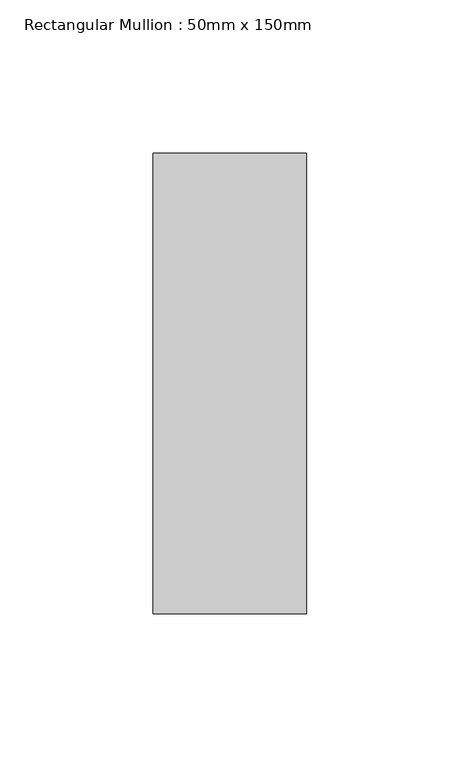
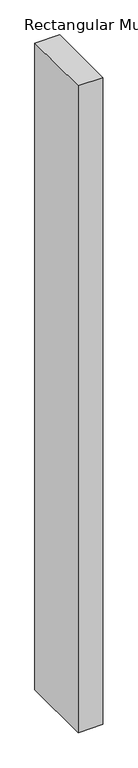
"""IFC4 building model written with IfcOpenShell, lengths in millimetres: member geometry, Rectangular Mullion : 50mm x 150mm."""

from ifc_helpers import new_model, si_unit, frame, origin, place, context, project, spatial, polyline, outline, extrude, source, transform, mapped, element, save


def rectangular_mullion_50mm_x_150mm_89a65e42(model_context):
    return source(origin(), model_context, "Body", "SweptSolid", [
        extrude(outline(polyline([(0.0, 75.0), (0.0, -75.0), (-50.0, -75.0), (-50.0, 75.0), (0.0, 75.0)])), frame((0.0, 0.0, -1374.5), z_axis=(0.0, 0.0, 1.0), x_axis=(1.0, 0.0, 0.0)), (0.0, 0.0, 1.0), 1374.5),
    ])


if __name__ == "__main__":
    model = new_model("IFC4")
    model_context = context("Model", 3, world=origin())
    ifc_project = project(units=[si_unit("LENGTHUNIT", "METRE", prefix="MILLI")], contexts=[model_context])
    site = spatial("IfcSite", under=ifc_project)
    building = spatial("IfcBuilding", under=site)
    placement = place(None, origin())
    rectangular_mullion_50mm_x_150mm_shape = rectangular_mullion_50mm_x_150mm_89a65e42(model_context)
    element("IfcMember", 1, ObjectType="Rectangular Mullion : 50mm x 150mm", at=placement, inside=building, context=model_context, shape_type="MappedRepresentation", body=[
        mapped(rectangular_mullion_50mm_x_150mm_shape, transform((0.0, 0.0, 0.0), x_axis=(1.0, 0.0, 0.0), y_axis=(0.0, 1.0, 0.0), z_axis=(0.0, 0.0, 1.0))),
    ])
    save(model, "model.ifc")

# Revit data of these elements
# Type "Rectangular Mullion : 50mm x 150mm"
#   built-in parameter 1007304 = 0.492126 (stored number, unit not read)
#   built-in parameter 1007301 = 0.082021 (stored number, unit not read)
#   built-in parameter 1007300 = 0.082021 (stored number, unit not read)
# Element 1 (IfcMember, "Rectangular Mullion : 50mm x 150mm")
#   Materials on its faces: "Aluminum"
# Materials
#   "Aluminum": class "Metal", colour RGB 244 244 244, transparency 0, Description = "Aluminum 6061", Cost = 0
